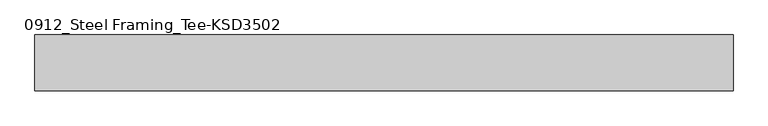
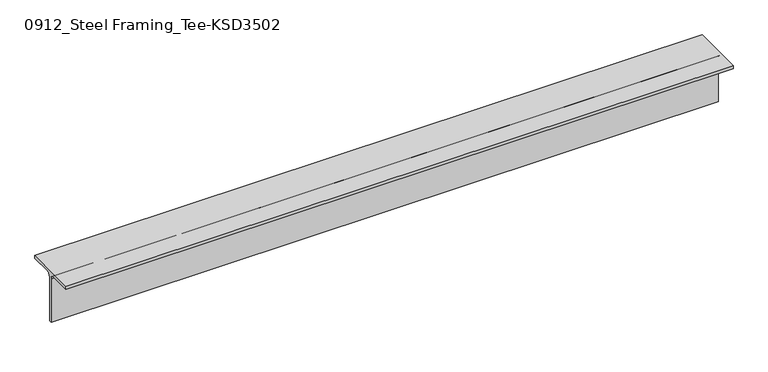
"""IFC4 building model written with IfcOpenShell, lengths in millimetres: member geometry, 0912_Steel Framing_Tee-KSD3502 : H_SB_ASB_CT-150x150x6.5x9."""

from ifc_helpers import new_model, si_unit, point, frame, frame_2d, origin, place, context, project, spatial, polyline, circle_curve, trimmed, segment, composite_curve, outline, extrude, source, transform, mapped, element, save


def member_0912_steel_framing_tee_ksd3502_d420d3ce(model_context):
    return source(origin(), model_context, "Body", "SweptSolid", [
        extrude(outline(composite_curve([segment(polyline([(-75.0, 75.0), (75.0, 75.0), (75.0, 66.0), (16.25, 66.0)]), True, "CONTINUOUS"), segment(trimmed(circle_curve(frame_2d((16.25, 53.0)), 13.0), [point((16.25, 66.0))], [point((3.25, 53.0))], True, "CARTESIAN"), True, "CONTINUOUS"), segment(polyline([(3.25, 53.0), (3.25, -75.0), (-3.25, -75.0), (-3.25, 53.0)]), True, "CONTINUOUS"), segment(trimmed(circle_curve(frame_2d((-16.25, 53.0)), 13.0), [point((-3.25, 53.0))], [point((-16.25, 66.0))], True, "CARTESIAN"), True, "CONTINUOUS"), segment(polyline([(-16.25, 66.0), (-75.0, 66.0), (-75.0, 75.0)]), True, "CONTINUOUS")], self_intersect=False)), frame((-1113.65, 0.0, 0.0), z_axis=(1.0, 0.0, 0.0), x_axis=(0.0, 1.0, 0.0)), (0.0, 0.0, 1.0), 1868.9),
    ])


if __name__ == "__main__":
    model = new_model("IFC4")
    model_context = context("Model", 3, world=origin())
    ifc_project = project(units=[si_unit("LENGTHUNIT", "METRE", prefix="MILLI")], contexts=[model_context])
    site = spatial("IfcSite", under=ifc_project)
    building = spatial("IfcBuilding", under=site)
    placement = place(None, origin())
    member_0912_steel_framing_tee_ksd3502_shape = member_0912_steel_framing_tee_ksd3502_d420d3ce(model_context)
    element("IfcMember", 1, ObjectType="0912_Steel Framing_Tee-KSD3502 : H_SB_ASB_CT-150x150x6.5x9", at=placement, inside=building, context=model_context, shape_type="MappedRepresentation", body=[
        mapped(member_0912_steel_framing_tee_ksd3502_shape, transform((0.0, 0.0, 0.0), x_axis=(1.0, 0.0, 0.0), y_axis=(0.0, 1.0, 0.0), z_axis=(0.0, 0.0, 1.0))),
    ])
    save(model, "model.ifc")

# Revit data of these elements
# Type "0912_Steel Framing_Tee-KSD3502 : H_SB_ASB_CT-150x150x6.5x9"
#   H_WM Code_1 = "S01AA003-00001 | Main Steel Structure Fabrication Work | Shelter/Building | Light Steel - Standard (30KG/M>Weight) | Material: (   )"
#   H_WM Code_2 = "S03AA029-00001 | Main Steel Structure Erection Work | Shelter/Building | Light Steel (30KG/M>Weight) | Material: (   )"
#   H_WM Code_3 = "S01AA010-00001 | Main Steel Structure Fabrication Work | Shelter/Building | Steel Painting/Coating | for Non-Fireproofed Steel Surface, Surface Preparation, Primer, Second & Final Coat | Material: (   )"
#   H_Q'ty Cal Type Tag = "SB-Q2"
#   Width = 15.0 cm
#   Web Thickness = 0.65 cm
#   Web Fillet = 1.3 cm
#   Section Area = 23.39 cm²
#   Perimeter = 0.60 m²/m
#   Nominal Weight = 18.40 kgf/m
#   Height = 15.0 cm
#   Flange Thickness = 0.9 cm
#   Centroid Vertical = 7.5 cm
#   Centroid Horizontal = 7.5 cm
#   Length [instance default] = 1.5000 m
#   Structural Material [instance default] = Steel, 45-345
#   Warping Constant = (empty or 0)
#   Torsional Moment of Inertia = 0
#   Section Name Key = ""
#   Plastic Modulus weak axis = 0
#   Plastic Modulus strong axis = 0
#   Moment of Inertia weak axis = 0
#   Moment of Inertia strong axis = 0
#   Elastic Modulus weak axis = 0
#   Elastic Modulus strong axis = 0
#   Bolt Spacing = 0
#   Assembly Code = ""
# Element 1 (IfcMember, "0912_Steel Framing_Tee-KSD3502 : H_SB_ASB_CT-150x150x6.5x9")
#   Structural Material = none
# Materials
#   "Steel, 45-345": class "Metal", colour RGB 189 187 185, transparency 0, Description = "Steel 345 MPa", Cost = 0
